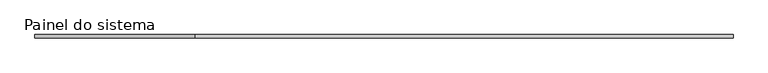
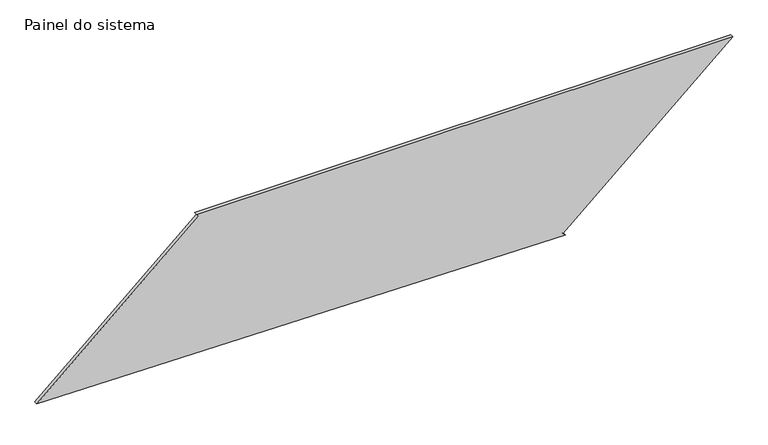
"""IFC4 building model written with IfcOpenShell, lengths in millimetres: plate geometry, Painel do sistema : Envidraçado."""

from ifc_helpers import new_model, si_unit, frame, origin, place, context, project, spatial, polyline, outline, extrude, source, transform, mapped, element, save


def painel_do_sistema_89c0715c(model_context):
    return source(origin(), model_context, "Body", "SweptSolid", [
        extrude(outline(polyline([(0.0, 1302.284687), (18.8079041, 1285.814631), (1090.2966682, 2509.3962658), (1090.2966682, -1357.6654943), (1071.488764, -1341.1954384), (48.4968973, -2509.3962658), (0.0, 1302.284687)])), frame((0.0, 24.5, 0.0), z_axis=(0.0, 1.0, 0.0), x_axis=(0.0, 0.0, 1.0)), (0.0, 0.0, 1.0), 25.0),
    ])


if __name__ == "__main__":
    model = new_model("IFC4")
    model_context = context("Model", 3, world=origin())
    ifc_project = project(units=[si_unit("LENGTHUNIT", "METRE", prefix="MILLI")], contexts=[model_context])
    site = spatial("IfcSite", under=ifc_project)
    building = spatial("IfcBuilding", under=site)
    placement = place(None, origin())
    painel_do_sistema_shape = painel_do_sistema_89c0715c(model_context)
    element("IfcPlate", 1, ObjectType="Painel do sistema : Envidraçado", at=placement, inside=building, context=model_context, shape_type="MappedRepresentation", body=[
        mapped(painel_do_sistema_shape, transform((0.0, 0.0, 0.0), x_axis=(1.0, 0.0, 0.0), y_axis=(0.0, 1.0, 0.0), z_axis=(0.0, 0.0, 1.0))),
    ])
    save(model, "model.ifc")

# Revit data of these elements
# Type "Painel do sistema : Envidraçado"
#   Construction Type Id = "GSP4R"
#   Analytic Construction = "Vidraça única Pilkington 1/8 pol"
#   Visual Light Transmittance = 0.9
#   Solar Heat Gain Coefficient = 0.86
#   Heat Transfer Coefficient (U) = 6.7069 W/(m²·K)
# Element 1 (IfcPlate, "Painel do sistema : Envidraçado")
#   Materials on its faces: "Vidro"
# Materials
#   "Vidro": class "Vidro", colour RGB 0 128 192, transparency 0.9, Description = "Vidro de sílica", Cost = 0
